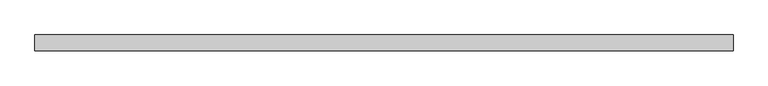
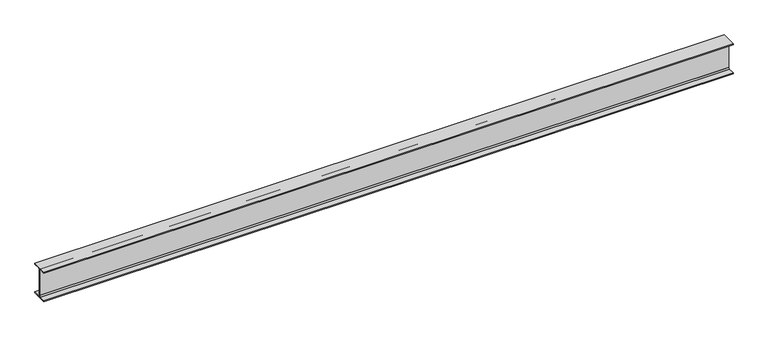
"""IFC4 building model written with IfcOpenShell, lengths in millimetres: beam geometry, 0912_Steel Framing_H-KSD3502 : H_SB_ASB_H-350x175x7x11."""

from ifc_helpers import new_model, si_unit, point, frame, frame_2d, origin, place, context, project, spatial, polyline, circle_curve, trimmed, segment, composite_curve, outline, extrude, source, transform, mapped, element, save


def beam_a6d55a04(model_context):
    return source(origin(), model_context, "Body", "SweptSolid", [
        extrude(outline(composite_curve([segment(polyline([(87.5, -164.0), (87.5, -175.0), (-87.5, -175.0), (-87.5, -164.0), (-17.5, -164.0)]), True, "CONTINUOUS"), segment(trimmed(circle_curve(frame_2d((-17.5, -150.0)), 14.0), [point((-17.5, -164.0))], [point((-3.5, -150.0))], True, "CARTESIAN"), True, "CONTINUOUS"), segment(polyline([(-3.5, -150.0), (-3.5, 150.0)]), True, "CONTINUOUS"), segment(trimmed(circle_curve(frame_2d((-17.5, 150.0)), 14.0), [point((-3.5, 150.0))], [point((-17.5, 164.0))], True, "CARTESIAN"), True, "CONTINUOUS"), segment(polyline([(-17.5, 164.0), (-87.5, 164.0), (-87.5, 175.0), (87.5, 175.0), (87.5, 164.0), (17.5, 164.0)]), True, "CONTINUOUS"), segment(trimmed(circle_curve(frame_2d((17.5, 150.0)), 14.0), [point((17.5, 164.0))], [point((3.5, 150.0))], True, "CARTESIAN"), True, "CONTINUOUS"), segment(polyline([(3.5, 150.0), (3.5, -150.0)]), True, "CONTINUOUS"), segment(trimmed(circle_curve(frame_2d((17.5, -150.0)), 14.0), [point((3.5, -150.0))], [point((17.5, -164.0))], True, "CARTESIAN"), True, "CONTINUOUS"), segment(polyline([(17.5, -164.0), (87.5, -164.0)]), True, "CONTINUOUS")], self_intersect=False)), frame((-3837.3, 0.0, 0.0), z_axis=(1.0, 0.0, 0.0), x_axis=(0.0, 1.0, 0.0)), (0.0, 0.0, 1.0), 7674.6),
    ])


if __name__ == "__main__":
    model = new_model("IFC4")
    model_context = context("Model", 3, world=origin())
    ifc_project = project(units=[si_unit("LENGTHUNIT", "METRE", prefix="MILLI")], contexts=[model_context])
    site = spatial("IfcSite", under=ifc_project)
    building = spatial("IfcBuilding", under=site)
    placement = place(None, origin())
    beam_shape = beam_a6d55a04(model_context)
    element("IfcBeam", 1, ObjectType="0912_Steel Framing_H-KSD3502 : H_SB_ASB_H-350x175x7x11", at=placement, inside=building, context=model_context, shape_type="MappedRepresentation", body=[
        mapped(beam_shape, transform((0.0, 0.0, 0.0), x_axis=(1.0, 0.0, 0.0), y_axis=(0.0, 1.0, 0.0), z_axis=(0.0, 0.0, 1.0))),
    ])
    save(model, "model.ifc")

# Revit data of these elements
# Type "0912_Steel Framing_H-KSD3502 : H_SB_ASB_H-350x175x7x11"
#   H_WM Code_1 = "S01AA002-00001 | Main Steel Structure Fabrication Work | Shelter/Building | Medium Steel - Standard (90KG/M>Weight≥30KG/M) | Material: (   )"
#   H_WM Code_2 = "S03AA028-00001 | Main Steel Structure Erection Work | Shelter/Building | Medium Steel (90KG/M>Weight≥30KG/M) | Material: (   )"
#   H_WM Code_3 = "S01AA010-00001 | Main Steel Structure Fabrication Work | Shelter/Building | Steel Painting/Coating | for Non-Fireproofed Steel Surface, Surface Preparation, Primer, Second & Final Coat | Material: (   )"
#   H_Q'ty Cal Type Tag = "SB-Q2"
#   Width = 17.5 cm
#   Web Thickness = 0.7 cm
#   Web Fillet = 1.4 cm
#   Warping Constant = 282000.0 cm⁶
#   W = 0
#   Torsional Moment of Inertia = 19.4042 cm⁴
#   Section Area = 63.14 cm²
#   Plastic Modulus weak axis = 174.0 cm³
#   Plastic Modulus strong axis = 868.0 cm³
#   Perimeter = 1.36 m²/m
#   Nominal Weight = 49.60 kgf/m
#   Moment of Inertia weak axis = 984.00 cm⁴
#   Moment of Inertia strong axis = 13600.00 cm⁴
#   Height = 35.0 cm
#   Flange Thickness = 1.1 cm
#   Elastic Modulus weak axis = 112.0 cm³
#   Elastic Modulus strong axis = 775.0 cm³
#   Centroid Vertical = 17.5 cm
#   Centroid Horizontal = 8.75 cm
#   Ix = 136000000
#   Length [instance default] = 1.5240 m
#   Zx = 868000
#   b = 0.1750 m
#   h = 0.3500 m
#   r = 0.0140 m
#   s = 0.0070 m
#   t = 0.0110 m
#   A = 0.006314 m²
#   Structural Material [instance default] = Steel, 45-345
#   Assembly Code = ""
# Element 1 (IfcBeam, "0912_Steel Framing_H-KSD3502 : H_SB_ASB_H-350x175x7x11")
#   Structural Material = none
# Materials
#   "Steel, 45-345": class "Metal", colour RGB 189 187 185, transparency 0, Description = "Steel 345 MPa", Cost = 0
